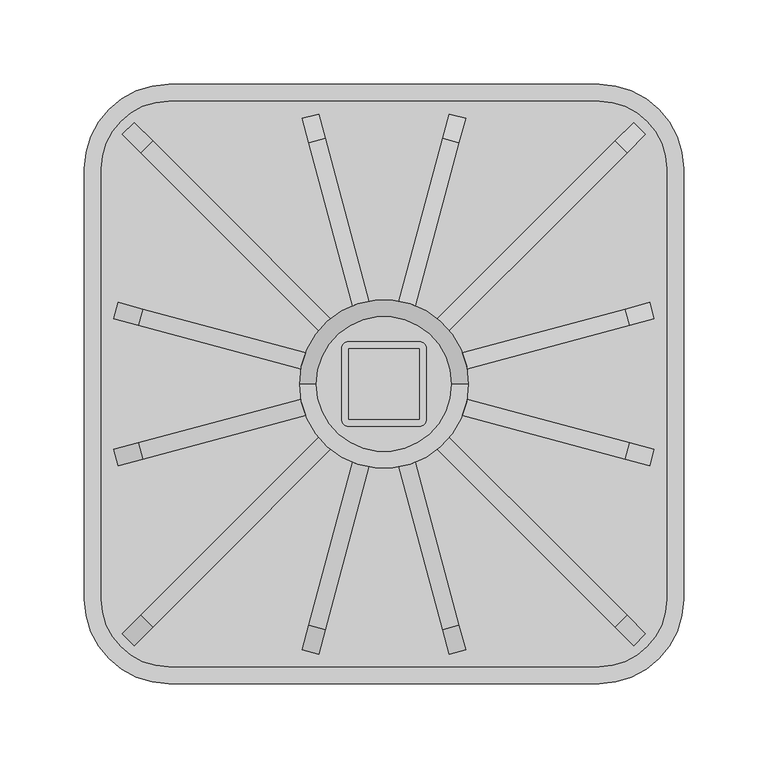
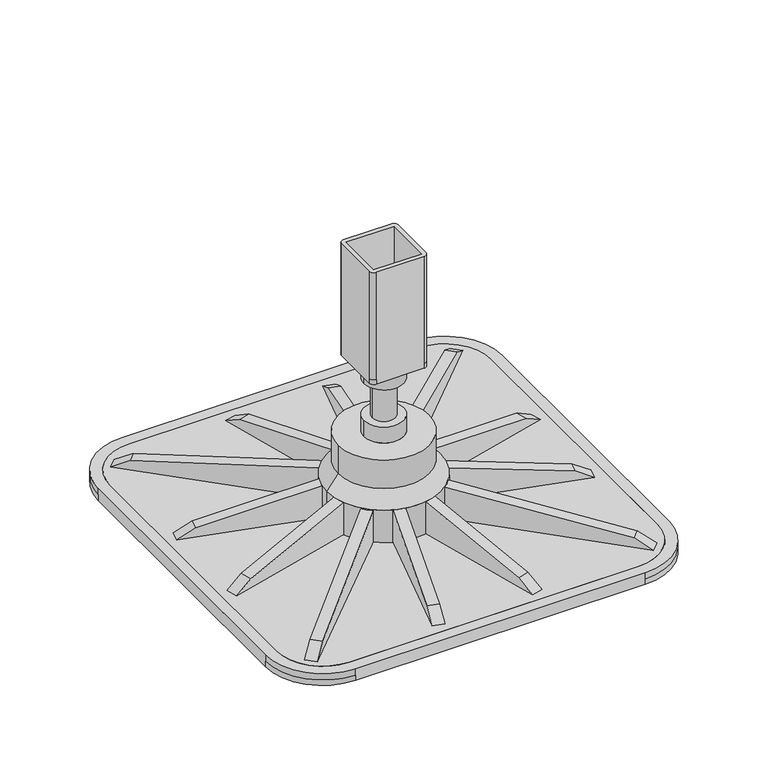
"""IFC4 building model written with IfcOpenShell, lengths in millimetres: proxy geometry, TN_Кровельная опора ТехноНИКОЛЬ : Кровельная опора ТехноНИКОЛЬ 355х355мм с вертикальным кронштейном."""

from ifc_helpers import new_model, si_unit, point, frame, frame_2d, origin, origin_2d, place, context, project, spatial, polyline, circle_curve, trimmed, segment, composite_curve, outline, extrude, source, transform, mapped, element, save
from ifc_brep_helpers import plane_surface, cylinder_surface, revolved_surface, advanced_brep


def generic_models_a60a2459(model_context):
    return source(origin(), model_context, "Body", "SolidModel", [
        extrude(outline(polyline([(214.1306058, 0.0), (198.8913097, -8.6706701), (0.0, -35.5445162), (0.0, 0.0), (214.1306058, 0.0)])), frame((-3.5355339, -3.5355339, 11.0), z_axis=(0.7071067811865469, 0.7071067811865482, 0.0), x_axis=(0.7071067811865482, -0.7071067811865469, 0.0)), (0.0, 0.0, 1.0), 10.0),
        extrude(outline(polyline([(0.0, 0.0), (17.5333016, 1e-07), (203.6920691, -74.9991329), (186.1143887, -105.8931094), (0.0, 0.0)])), frame((154.9487373, 147.8776695, 11.0), z_axis=(-0.707106781186547, 0.7071067811865481, 0.0), x_axis=(-0.6145910150795418, -0.6145910150795407, 0.49452580151797754)), (0.0, 0.0, 1.0), 10.0),
        extrude(outline(polyline([(-214.1306058, 0.0), (0.0, 0.0), (0.0, -35.5445162), (-198.8913097, -8.6706701), (-214.1306058, 0.0)])), frame((-3.5355339, -3.5355339, 11.0), z_axis=(0.7071067811865469, 0.7071067811865482, 0.0), x_axis=(0.7071067811865482, -0.7071067811865469, 0.0)), (0.0, 0.0, 1.0), 10.0),
        extrude(outline(polyline([(0.0, 0.0), (-142.9576707, -80.9713708), (-162.6162897, -46.2634197), (-17.1780129, 0.0), (0.0, 0.0)])), frame((-38.6654497, -159.9920884, 11.0), z_axis=(-0.9659258262890678, 0.25881904510252296, 0.0), x_axis=(-0.22520396734385073, -0.8404726481933256, -0.4928376007687403)), (0.0, 0.0, 1.0), 10.0),
        extrude(outline(polyline([(164.4678969, 0.0), (149.5209418, -8.4659707), (0.1716447, -39.8886346), (0.1716447, 0.0), (164.4678969, 0.0)])), frame((-3.9019744, -1.1282992, 11.0), z_axis=(0.9659258262890678, 0.25881904510252296, 0.0), x_axis=(0.25881904510252296, -0.9659258262890678, 0.0)), (0.0, 0.0, 1.0), 10.0),
        extrude(outline(polyline([(0.0, 0.0), (17.1780129, 0.0), (162.6162896, -46.2634196), (142.9576706, -80.9713707), (0.0, 0.0)])), frame((157.4038979, -48.3247079, 11.0), z_axis=(0.2588190451025272, 0.9659258262890665, 0.0), x_axis=(-0.8404726481933232, 0.22520396734385406, 0.4928376007687429)), (0.0, 0.0, 1.0), 10.0),
        extrude(outline(polyline([(164.4678969, 0.0), (149.5209418, -8.4659707), (0.1716447, -39.8886346), (0.1716447, 0.0), (164.4678969, 0.0)])), frame((1.1282992, -3.9019744, 11.0), z_axis=(-0.25881904510252723, 0.9659258262890665, 0.0), x_axis=(0.9659258262890665, 0.25881904510252723, 0.0)), (0.0, 0.0, 1.0), 10.0),
        extrude(outline(polyline([(0.0, 0.0), (17.1780129, 0.0), (162.6162896, -46.2634196), (142.9576706, -80.9713707), (0.0, 0.0)])), frame((48.3247079, 157.4038979, 11.0), z_axis=(-0.9659258262890661, 0.2588190451025289, 0.0), x_axis=(-0.22520396734385595, -0.8404726481933242, 0.4928376007687402)), (0.0, 0.0, 1.0), 10.0),
        extrude(outline(polyline([(-164.4678969, 0.0), (-0.1716447, 0.0), (-0.1716447, -39.8886346), (-149.5209418, -8.4659707), (-164.4678969, 0.0)])), frame((-5.7572839, -1.4598913, 11.0), z_axis=(0.9659258262890661, 0.25881904510252896, 0.0), x_axis=(0.25881904510252896, -0.9659258262890661, 0.0)), (0.0, 0.0, 1.0), 10.0),
        extrude(outline(polyline([(0.0, 0.0), (-142.9576707, -80.9713708), (-162.6162897, -46.2634197), (-17.1780129, 0.0), (0.0, 0.0)])), frame((-159.9920884, 38.6654497, 11.0), z_axis=(0.25881904510253323, 0.9659258262890649, 0.0), x_axis=(-0.8404726481933251, 0.2252039673438602, -0.4928376007687367)), (0.0, 0.0, 1.0), 10.0),
        extrude(outline(composite_curve([segment(trimmed(circle_curve(origin_2d(), 17.25), [point((-17.25, 0.0))], [point((17.25, 0.0))], False, "CARTESIAN"), True, "CONTINUOUS"), segment(trimmed(circle_curve(origin_2d(), 17.25), [point((17.25, 0.0))], [point((-17.25, 0.0))], False, "CARTESIAN"), True, "CONTINUOUS")], self_intersect=False)), frame((0.0, 0.0, 130.0), z_axis=(0.0, 0.0, 1.0), x_axis=(1.0, 0.0, 0.0)), (0.0, 0.0, 1.0), 16.0),
        advanced_brep(
        [(-21.0, 21.0, 150.0), (-21.0, -21.0, 150.0), (21.0, -21.0, 150.0), (21.0, 21.0, 150.0), (-25.0, 21.0, 146.0), (-21.0, 25.0, 146.0), (21.0, 25.0, 146.0), (25.0, 21.0, 146.0), (25.0, -21.0, 146.0), (21.0, -25.0, 146.0), (-21.0, -25.0, 146.0), (-25.0, -21.0, 146.0), (-25.0, -21.0, 150.0), (-25.0, -21.0, 250.0), (-25.0, 21.0, 250.0), (-25.0, 21.0, 150.0), (-21.0, -25.0, 150.0), (21.0, -25.0, 150.0), (21.0, -25.0, 250.0), (-21.0, -25.0, 250.0), (25.0, -21.0, 150.0), (25.0, 21.0, 150.0), (25.0, 21.0, 250.0), (25.0, -21.0, 250.0), (21.0, 25.0, 150.0), (-21.0, 25.0, 150.0), (-21.0, 25.0, 250.0), (21.0, 25.0, 250.0), (-21.0, -21.0, 250.0), (-21.0, 21.0, 250.0), (21.0, 21.0, 250.0), (21.0, -21.0, 250.0)],
        [
            (0, 1),
            (1, 2),
            (2, 3),
            (3, 0),
            (4, 5, circle_curve(frame((-21.0, 21.0, 146.0), z_axis=(0.0, 0.0, -1.0), x_axis=(1.0, 0.0, 0.0)), 4.0)),
            (5, 6),
            (6, 7, circle_curve(frame((21.0, 21.0, 146.0), z_axis=(0.0, 0.0, -1.0), x_axis=(1.0, 0.0, 0.0)), 4.0)),
            (7, 8),
            (8, 9, circle_curve(frame((21.0, -21.0, 146.0), z_axis=(0.0, 0.0, -1.0), x_axis=(1.0, 0.0, 0.0)), 4.0)),
            (9, 10),
            (10, 11, circle_curve(frame((-21.0, -21.0, 146.0), z_axis=(0.0, 0.0, -1.0), x_axis=(1.0, 0.0, 0.0)), 4.0)),
            (11, 4),
            (11, 12),
            (12, 13),
            (13, 14),
            (14, 15),
            (15, 4),
            (10, 16),
            (16, 12, circle_curve(frame((-21.0, -21.0, 150.0), z_axis=(0.0, 0.0, -1.0), x_axis=(1.0, 0.0, 0.0)), 4.0)),
            (9, 17),
            (17, 18),
            (18, 19),
            (19, 16),
            (8, 20),
            (20, 17, circle_curve(frame((21.0, -21.0, 150.0), z_axis=(0.0, 0.0, -1.0), x_axis=(1.0, 0.0, 0.0)), 4.0)),
            (7, 21),
            (21, 22),
            (22, 23),
            (23, 20),
            (6, 24),
            (24, 21, circle_curve(frame((21.0, 21.0, 150.0), z_axis=(0.0, 0.0, -1.0), x_axis=(1.0, 0.0, 0.0)), 4.0)),
            (5, 25),
            (25, 26),
            (26, 27),
            (27, 24),
            (15, 25, circle_curve(frame((-21.0, 21.0, 150.0), z_axis=(0.0, 0.0, -1.0), x_axis=(1.0, 0.0, 0.0)), 4.0)),
            (26, 14, circle_curve(frame((-21.0, 21.0, 250.0), z_axis=(0.0, 0.0, 1.0), x_axis=(1.0, 0.0, 0.0)), 4.0)),
            (13, 19, circle_curve(frame((-21.0, -21.0, 250.0), z_axis=(0.0, 0.0, 1.0), x_axis=(1.0, 0.0, 0.0)), 4.0)),
            (18, 23, circle_curve(frame((21.0, -21.0, 250.0), z_axis=(0.0, 0.0, 1.0), x_axis=(1.0, 0.0, 0.0)), 4.0)),
            (22, 27, circle_curve(frame((21.0, 21.0, 250.0), z_axis=(0.0, 0.0, 1.0), x_axis=(1.0, 0.0, 0.0)), 4.0)),
            (28, 29),
            (29, 30),
            (30, 31),
            (31, 28),
            (28, 1),
            (0, 29),
            (3, 30),
            (2, 31),
        ],
        [
            plane_surface(frame((-25.0, 21.0, 150.0), z_axis=(0.0, 0.0, 1.0), x_axis=(0.0, -1.0, 0.0))),
            plane_surface(frame((-25.0, 21.0, 146.0), z_axis=(0.0, 0.0, -1.0), x_axis=(0.0, 1.0, 0.0))),
            plane_surface(frame((-25.0, 21.0, 150.0), z_axis=(-1.0, 0.0, 0.0), x_axis=(0.0, 0.0, -1.0))),
            cylinder_surface(frame((-21.0, -21.0, 146.0), z_axis=(0.0, 0.0, 1.0), x_axis=(1.0, 0.0, 0.0)), 4.0),
            plane_surface(frame((-21.0, -25.0, 150.0), z_axis=(0.0, -1.0, 0.0), x_axis=(0.0, 0.0, -1.0))),
            cylinder_surface(frame((21.0, -21.0, 146.0), z_axis=(0.0, 0.0, 1.0), x_axis=(1.0, 0.0, 0.0)), 4.0),
            plane_surface(frame((25.0, -21.0, 150.0), z_axis=(1.0, 0.0, 0.0), x_axis=(0.0, 0.0, -1.0))),
            cylinder_surface(frame((21.0, 21.0, 146.0), z_axis=(0.0, 0.0, 1.0), x_axis=(1.0, 0.0, 0.0)), 4.0),
            plane_surface(frame((21.0, 25.0, 150.0), z_axis=(0.0, 1.0, 0.0), x_axis=(0.0, 0.0, -1.0))),
            cylinder_surface(frame((-21.0, 21.0, 146.0), z_axis=(0.0, 0.0, 1.0), x_axis=(1.0, 0.0, 0.0)), 4.0),
            plane_surface(frame((-25.0, 25.0, 250.0), z_axis=(0.0, 0.0, 1.0), x_axis=(-1.0, 0.0, 0.0))),
            plane_surface(frame((-21.0, -21.0, 250.0), z_axis=(1.0, 0.0, 0.0), x_axis=(0.0, 0.0, -1.0))),
            plane_surface(frame((-21.0, 21.0, 250.0), z_axis=(0.0, -1.0, 0.0), x_axis=(0.0, 0.0, -1.0))),
            plane_surface(frame((21.0, 21.0, 250.0), z_axis=(-1.0, 0.0, 0.0), x_axis=(0.0, 0.0, -1.0))),
            plane_surface(frame((21.0, -21.0, 250.0), z_axis=(0.0, 1.0, 0.0), x_axis=(0.0, 0.0, -1.0))),
        ],
        [
            (0, [[1, 2, 3, 4]]),
            (1, [[5, 6, 7, 8, 9, 10, 11, 12]]),
            (2, [[-12, 13, 14, 15, 16, 17]]),
            (3, [[-11, 18, 19, -13]]),
            (4, [[-10, 20, 21, 22, 23, -18]]),
            (5, [[-9, 24, 25, -20]]),
            (6, [[-8, 26, 27, 28, 29, -24]]),
            (7, [[-7, 30, 31, -26]]),
            (8, [[-6, 32, 33, 34, 35, -30]]),
            (9, [[-5, -17, 36, -32]]),
            (10, [[-34, 37, -15, 38, -22, 39, -28, 40], [41, 42, 43, 44]]),
            (9, [[-37, -33, -36, -16]]),
            (3, [[-38, -14, -19, -23]]),
            (5, [[-39, -21, -25, -29]]),
            (7, [[-40, -27, -31, -35]]),
            (11, [[-41, 45, -1, 46]]),
            (12, [[-42, -46, -4, 47]]),
            (13, [[-43, -47, -3, 48]]),
            (14, [[-44, -48, -2, -45]]),
        ],
    ),
        advanced_brep(
        [(-40.0, 0.0, 80.6), (40.0, 0.0, 80.6), (17.25, 0.0, 80.6), (-17.25, 0.0, 80.6), (-40.0, 0.0, 54.2), (40.0, 0.0, 54.2), (-10.0, 0.0, 146.0), (10.0, 0.0, 146.0), (-10.0, 0.0, 95.6), (10.0, 0.0, 95.6), (-17.25, 0.0, 95.6), (17.25, 0.0, 95.6)],
        [
            (0, 1, circle_curve(frame((0.0, 0.0, 80.6), z_axis=(0.0, 0.0, 1.0), x_axis=(1.0, 0.0, 0.0)), 40.0)),
            (1, 0, circle_curve(frame((0.0, 0.0, 80.6), z_axis=(0.0, 0.0, 1.0), x_axis=(1.0, 0.0, 0.0)), 40.0)),
            (2, 3, circle_curve(frame((0.0, 0.0, 80.6), z_axis=(0.0, 0.0, -1.0), x_axis=(1.0, 0.0, 0.0)), 17.25)),
            (3, 2, circle_curve(frame((0.0, 0.0, 80.6), z_axis=(0.0, 0.0, -1.0), x_axis=(1.0, 0.0, 0.0)), 17.25)),
            (4, 5, circle_curve(frame((0.0, 0.0, 54.2), z_axis=(0.0, 0.0, -1.0), x_axis=(1.0, 0.0, 0.0)), 40.0)),
            (5, 4, circle_curve(frame((0.0, 0.0, 54.2), z_axis=(0.0, 0.0, -1.0), x_axis=(1.0, 0.0, 0.0)), 40.0)),
            (0, 4),
            (5, 1),
            (6, 7, circle_curve(frame((0.0, 0.0, 146.0), z_axis=(0.0, 0.0, 1.0), x_axis=(1.0, 0.0, 0.0)), 10.0)),
            (7, 6, circle_curve(frame((0.0, 0.0, 146.0), z_axis=(0.0, 0.0, 1.0), x_axis=(1.0, 0.0, 0.0)), 10.0)),
            (6, 8),
            (8, 9, circle_curve(frame((0.0, 0.0, 95.6), z_axis=(0.0, 0.0, 1.0), x_axis=(1.0, 0.0, 0.0)), 10.0)),
            (9, 7),
            (9, 8, circle_curve(frame((0.0, 0.0, 95.6), z_axis=(0.0, 0.0, 1.0), x_axis=(1.0, 0.0, 0.0)), 10.0)),
            (10, 11, circle_curve(frame((0.0, 0.0, 95.6), z_axis=(0.0, 0.0, 1.0), x_axis=(1.0, 0.0, 0.0)), 17.25)),
            (11, 10, circle_curve(frame((0.0, 0.0, 95.6), z_axis=(0.0, 0.0, 1.0), x_axis=(1.0, 0.0, 0.0)), 17.25)),
            (10, 3),
            (2, 11),
        ],
        [
            plane_surface(frame((40.0, 0.0, 80.6), z_axis=(0.0, 0.0, 1.0), x_axis=(0.0, 1.0, 0.0))),
            plane_surface(frame((40.0, 0.0, 54.2), z_axis=(0.0, 0.0, -1.0), x_axis=(0.0, -1.0, 0.0))),
            cylinder_surface(frame((0.0, 0.0, 54.2), z_axis=(0.0, 0.0, 1.0), x_axis=(1.0, 0.0, 0.0)), 40.0),
            plane_surface(frame((10.0, 0.0, 146.0), z_axis=(0.0, 0.0, 1.0), x_axis=(0.0, 1.0, 0.0))),
            cylinder_surface(frame((0.0, 0.0, 80.6), z_axis=(0.0, 0.0, 1.0), x_axis=(1.0, 0.0, 0.0)), 10.0),
            plane_surface(frame((17.25, 0.0, 95.6), z_axis=(0.0, 0.0, 1.0), x_axis=(0.0, 1.0, 0.0))),
            cylinder_surface(frame((0.0, 0.0, 80.6), z_axis=(0.0, 0.0, 1.0), x_axis=(1.0, 0.0, 0.0)), 17.25),
        ],
        [
            (0, [[1, 2], [3, 4]]),
            (1, [[5, 6]]),
            (2, [[-1, 7, -6, 8]]),
            (2, [[-2, -8, -5, -7]]),
            (3, [[9, 10]]),
            (4, [[-9, 11, 12, 13]]),
            (4, [[-10, -13, 14, -11]]),
            (5, [[15, 16], [-12, -14]]),
            (6, [[-15, 17, -3, 18]]),
            (6, [[-16, -18, -4, -17]]),
        ],
    ),
        extrude(outline(polyline([(-164.4678969, 0.0), (-0.1716447, 0.0), (-0.1716447, -39.8886346), (-149.5209418, -8.4659707), (-164.4678969, 0.0)])), frame((1.4598913, -5.7572839, 11.0), z_axis=(-0.25881904510253323, 0.965925826289065, 0.0), x_axis=(0.965925826289065, 0.25881904510253323, 0.0)), (0.0, 0.0, 1.0), 10.0),
        extrude(outline(polyline([(0.0, 0.0), (-186.1143887, -105.8931094), (-203.6920691, -74.9991329), (-17.5333016, 1e-07), (0.0, 0.0)])), frame((-147.8776695, -154.9487373, 11.0), z_axis=(-0.7071067811865469, 0.7071067811865482, 0.0), x_axis=(-0.6145910150795192, -0.6145910150795181, -0.4945258015180338)), (0.0, 0.0, 1.0), 10.0),
        advanced_brep(
        [(-40.0, 0.0, 54.2), (40.0, 0.0, 54.2), (-50.0, 0.0, 41.0), (50.0, 0.0, 41.0)],
        [
            (0, 1, circle_curve(frame((0.0, 0.0, 54.2), z_axis=(0.0, 0.0, 1.0), x_axis=(-1.0, 0.0, 0.0)), 40.0)),
            (1, 0, circle_curve(frame((0.0, 0.0, 54.2), z_axis=(0.0, 0.0, 1.0), x_axis=(1.0, 0.0, 0.0)), 40.0)),
            (2, 3, circle_curve(frame((0.0, 0.0, 41.0), z_axis=(0.0, 0.0, -1.0), x_axis=(1.0, 0.0, 0.0)), 50.0)),
            (3, 2, circle_curve(frame((0.0, 0.0, 41.0), z_axis=(0.0, 0.0, -1.0), x_axis=(-1.0, 0.0, 0.0)), 50.0)),
            (3, 1),
            (0, 2),
        ],
        [
            plane_surface(frame((0.0, 0.0, 54.2), z_axis=(0.0, 0.0, 1.0), x_axis=(0.0, -1.0, 0.0))),
            plane_surface(frame((0.0, 0.0, 41.0), z_axis=(0.0, 0.0, -1.0), x_axis=(0.0, -1.0, 0.0))),
            revolved_surface(polyline([(-40.0, 0.0, 54.2), (-50.0, 0.0, 41.0)]), (0.0, 0.0, 107.0), (0.0, 0.0, -1.0)),
            revolved_surface(polyline([(40.0, 0.0, 54.2), (50.0, 0.0, 41.0)]), (0.0, 0.0, 107.0), (0.0, 0.0, -1.0)),
        ],
        [
            (0, [[1, 2]]),
            (1, [[3, 4]]),
            (2, [[-4, 5, -1, 6]]),
            (3, [[-3, -6, -2, -5]]),
        ],
    ),
        extrude(outline(composite_curve([segment(trimmed(circle_curve(origin_2d(), 50.0), [point((-50.0, 0.0))], [point((50.0, 0.0))], False, "CARTESIAN"), True, "CONTINUOUS"), segment(trimmed(circle_curve(origin_2d(), 50.0), [point((50.0, 0.0))], [point((-50.0, 0.0))], False, "CARTESIAN"), True, "CONTINUOUS")], self_intersect=False)), frame((0.0, 0.0, 11.0), z_axis=(0.0, 0.0, 1.0), x_axis=(1.0, 0.0, 0.0)), (0.0, 0.0, 1.0), 30.0),
        extrude(outline(composite_curve([segment(trimmed(circle_curve(frame_2d((127.5, 127.5)), 40.0), [point((127.5, 167.5))], [point((167.5, 127.5))], False, "CARTESIAN"), True, "CONTINUOUS"), segment(polyline([(167.5, 127.5), (167.5, -127.5)]), True, "CONTINUOUS"), segment(trimmed(circle_curve(frame_2d((127.5, -127.5)), 40.0), [point((167.5, -127.5))], [point((127.5, -167.5))], False, "CARTESIAN"), True, "CONTINUOUS"), segment(polyline([(127.5, -167.5), (-127.5, -167.5)]), True, "CONTINUOUS"), segment(trimmed(circle_curve(frame_2d((-127.5, -127.5)), 40.0), [point((-127.5, -167.5))], [point((-167.5, -127.5))], False, "CARTESIAN"), True, "CONTINUOUS"), segment(polyline([(-167.5, -127.5), (-167.5, 127.5)]), True, "CONTINUOUS"), segment(trimmed(circle_curve(frame_2d((-127.5, 127.5)), 40.0), [point((-167.5, 127.5))], [point((-127.5, 167.5))], False, "CARTESIAN"), True, "CONTINUOUS"), segment(polyline([(-127.5, 167.5), (127.5, 167.5)]), True, "CONTINUOUS")], self_intersect=False)), frame((0.0, 0.0, 5.0), z_axis=(0.0, 0.0, 1.0), x_axis=(1.0, 0.0, 0.0)), (0.0, 0.0, 1.0), 6.0),
        advanced_brep(
        [(-127.5, 167.5, 5.0), (-167.5, 127.5, 5.0), (-167.5, -127.5, 5.0), (-127.5, -167.5, 5.0), (127.5, -167.5, 5.0), (167.5, -127.5, 5.0), (167.5, 127.5, 5.0), (127.5, 167.5, 5.0), (-177.5, -127.5, 0.0), (-177.5, 127.5, 0.0), (-127.5, 177.5, 0.0), (127.5, 177.5, 0.0), (177.5, 127.5, 0.0), (177.5, -127.5, 0.0), (127.5, -177.5, 0.0), (-127.5, -177.5, 0.0), (-127.5, -177.5, 5.0), (-177.5, -127.5, 5.0), (127.5, -177.5, 5.0), (127.5, -177.5, 11.0), (-127.5, -177.5, 11.0), (177.5, -127.5, 5.0), (177.5, 127.5, 5.0), (177.5, 127.5, 11.0), (177.5, -127.5, 11.0), (127.5, 177.5, 5.0), (-127.5, 177.5, 5.0), (-127.5, 177.5, 11.0), (127.5, 177.5, 11.0), (-177.5, 127.5, 5.0), (-177.5, -127.5, 11.0), (-177.5, 127.5, 11.0), (-167.5, 127.5, 11.0), (-127.5, 167.5, 11.0), (127.5, 167.5, 11.0), (167.5, 127.5, 11.0), (167.5, -127.5, 11.0), (127.5, -167.5, 11.0), (-127.5, -167.5, 11.0), (-167.5, -127.5, 11.0)],
        [
            (0, 1, circle_curve(frame((-127.5, 127.5, 5.0), z_axis=(0.0, 0.0, 1.0), x_axis=(1.0, 0.0, 0.0)), 40.0)),
            (1, 2),
            (2, 3, circle_curve(frame((-127.5, -127.5, 5.0), z_axis=(0.0, 0.0, 1.0), x_axis=(1.0, 0.0, 0.0)), 40.0)),
            (3, 4),
            (4, 5, circle_curve(frame((127.5, -127.5, 5.0), z_axis=(0.0, 0.0, 1.0), x_axis=(1.0, 0.0, 0.0)), 40.0)),
            (5, 6),
            (6, 7, circle_curve(frame((127.5, 127.5, 5.0), z_axis=(0.0, 0.0, 1.0), x_axis=(1.0, 0.0, 0.0)), 40.0)),
            (7, 0),
            (8, 9),
            (9, 10, circle_curve(frame((-127.5, 127.5, 0.0), z_axis=(0.0, 0.0, -1.0), x_axis=(1.0, 0.0, 0.0)), 50.0)),
            (10, 11),
            (11, 12, circle_curve(frame((127.5, 127.5, 0.0), z_axis=(0.0, 0.0, -1.0), x_axis=(1.0, 0.0, 0.0)), 50.0)),
            (12, 13),
            (13, 14, circle_curve(frame((127.5, -127.5, 0.0), z_axis=(0.0, 0.0, -1.0), x_axis=(1.0, 0.0, 0.0)), 50.0)),
            (14, 15),
            (15, 8, circle_curve(frame((-127.5, -127.5, 0.0), z_axis=(0.0, 0.0, -1.0), x_axis=(1.0, 0.0, 0.0)), 50.0)),
            (15, 16),
            (16, 17, circle_curve(frame((-127.5, -127.5, 5.0), z_axis=(0.0, 0.0, -1.0), x_axis=(1.0, 0.0, 0.0)), 50.0)),
            (17, 8),
            (14, 18),
            (18, 19),
            (19, 20),
            (20, 16),
            (13, 21),
            (21, 18, circle_curve(frame((127.5, -127.5, 5.0), z_axis=(0.0, 0.0, -1.0), x_axis=(1.0, 0.0, 0.0)), 50.0)),
            (12, 22),
            (22, 23),
            (23, 24),
            (24, 21),
            (11, 25),
            (25, 22, circle_curve(frame((127.5, 127.5, 5.0), z_axis=(0.0, 0.0, -1.0), x_axis=(1.0, 0.0, 0.0)), 50.0)),
            (10, 26),
            (26, 27),
            (27, 28),
            (28, 25),
            (9, 29),
            (29, 26, circle_curve(frame((-127.5, 127.5, 5.0), z_axis=(0.0, 0.0, -1.0), x_axis=(1.0, 0.0, 0.0)), 50.0)),
            (17, 30),
            (30, 31),
            (31, 29),
            (27, 31, circle_curve(frame((-127.5, 127.5, 11.0), z_axis=(0.0, 0.0, 1.0), x_axis=(1.0, 0.0, 0.0)), 50.0)),
            (30, 20, circle_curve(frame((-127.5, -127.5, 11.0), z_axis=(0.0, 0.0, 1.0), x_axis=(1.0, 0.0, 0.0)), 50.0)),
            (19, 24, circle_curve(frame((127.5, -127.5, 11.0), z_axis=(0.0, 0.0, 1.0), x_axis=(1.0, 0.0, 0.0)), 50.0)),
            (23, 28, circle_curve(frame((127.5, 127.5, 11.0), z_axis=(0.0, 0.0, 1.0), x_axis=(1.0, 0.0, 0.0)), 50.0)),
            (32, 33, circle_curve(frame((-127.5, 127.5, 11.0), z_axis=(0.0, 0.0, -1.0), x_axis=(1.0, 0.0, 0.0)), 40.0)),
            (33, 34),
            (34, 35, circle_curve(frame((127.5, 127.5, 11.0), z_axis=(0.0, 0.0, -1.0), x_axis=(1.0, 0.0, 0.0)), 40.0)),
            (35, 36),
            (36, 37, circle_curve(frame((127.5, -127.5, 11.0), z_axis=(0.0, 0.0, -1.0), x_axis=(1.0, 0.0, 0.0)), 40.0)),
            (37, 38),
            (38, 39, circle_curve(frame((-127.5, -127.5, 11.0), z_axis=(0.0, 0.0, -1.0), x_axis=(1.0, 0.0, 0.0)), 40.0)),
            (39, 32),
            (32, 1),
            (0, 33),
            (7, 34),
            (6, 35),
            (5, 36),
            (4, 37),
            (3, 38),
            (2, 39),
        ],
        [
            plane_surface(frame((-77.5, -127.5, 5.0), z_axis=(0.0, 0.0, 1.0), x_axis=(0.0, 1.0, 0.0))),
            plane_surface(frame((-77.5, -127.5, 0.0), z_axis=(0.0, 0.0, -1.0), x_axis=(0.0, -1.0, 0.0))),
            cylinder_surface(frame((-127.5, -127.5, 0.0), z_axis=(0.0, 0.0, 1.0), x_axis=(1.0, 0.0, 0.0)), 50.0),
            plane_surface(frame((-127.5, -177.5, 5.0), z_axis=(0.0, -1.0, 0.0), x_axis=(0.0, 0.0, -1.0))),
            cylinder_surface(frame((127.5, -127.5, 0.0), z_axis=(0.0, 0.0, 1.0), x_axis=(1.0, 0.0, 0.0)), 50.0),
            plane_surface(frame((177.5, -127.5, 5.0), z_axis=(1.0, 0.0, 0.0), x_axis=(0.0, 0.0, -1.0))),
            cylinder_surface(frame((127.5, 127.5, 0.0), z_axis=(0.0, 0.0, 1.0), x_axis=(1.0, 0.0, 0.0)), 50.0),
            plane_surface(frame((127.5, 177.5, 5.0), z_axis=(0.0, 1.0, 0.0), x_axis=(0.0, 0.0, -1.0))),
            cylinder_surface(frame((-127.5, 127.5, 0.0), z_axis=(0.0, 0.0, 1.0), x_axis=(1.0, 0.0, 0.0)), 50.0),
            plane_surface(frame((-177.5, 127.5, 5.0), z_axis=(-1.0, 0.0, 0.0), x_axis=(0.0, 0.0, -1.0))),
            plane_surface(frame((-77.5, 127.5, 11.0), z_axis=(0.0, 0.0, 1.0), x_axis=(0.0, 1.0, 0.0))),
            cylinder_surface(frame((-127.5, 127.5, 5.0), z_axis=(0.0, 0.0, 1.0), x_axis=(1.0, 0.0, 0.0)), 50.0),
            cylinder_surface(frame((-127.5, -127.5, 5.0), z_axis=(0.0, 0.0, 1.0), x_axis=(1.0, 0.0, 0.0)), 50.0),
            cylinder_surface(frame((127.5, -127.5, 5.0), z_axis=(0.0, 0.0, 1.0), x_axis=(1.0, 0.0, 0.0)), 50.0),
            cylinder_surface(frame((127.5, 127.5, 5.0), z_axis=(0.0, 0.0, 1.0), x_axis=(1.0, 0.0, 0.0)), 50.0),
            revolved_surface(polyline([(-87.5, 127.5, 5.0), (-87.5, 127.5, 11.0)]), (-127.5, 127.5, 0.0), (0.0, 0.0, -1.0)),
            plane_surface(frame((-127.5, 167.5, 11.0), z_axis=(0.0, -1.0, 0.0), x_axis=(0.0, 0.0, -1.0))),
            revolved_surface(polyline([(167.5, 127.5, 5.0), (167.5, 127.5, 11.0)]), (127.5, 127.5, 0.0), (0.0, 0.0, -1.0)),
            plane_surface(frame((167.5, 127.5, 11.0), z_axis=(-1.0, 0.0, 0.0), x_axis=(0.0, 0.0, -1.0))),
            revolved_surface(polyline([(167.5, -127.5, 5.0), (167.5, -127.5, 11.0)]), (127.5, -127.5, 0.0), (0.0, 0.0, -1.0)),
            plane_surface(frame((127.5, -167.5, 11.0), z_axis=(0.0, 1.0, 0.0), x_axis=(0.0, 0.0, -1.0))),
            revolved_surface(polyline([(-87.5, -127.5, 5.0), (-87.5, -127.5, 11.0)]), (-127.5, -127.5, 0.0), (0.0, 0.0, -1.0)),
            plane_surface(frame((-167.5, -127.5, 11.0), z_axis=(1.0, 0.0, 0.0), x_axis=(0.0, 0.0, -1.0))),
        ],
        [
            (0, [[1, 2, 3, 4, 5, 6, 7, 8]]),
            (1, [[9, 10, 11, 12, 13, 14, 15, 16]]),
            (2, [[-16, 17, 18, 19]]),
            (3, [[-15, 20, 21, 22, 23, -17]]),
            (4, [[-14, 24, 25, -20]]),
            (5, [[-13, 26, 27, 28, 29, -24]]),
            (6, [[-12, 30, 31, -26]]),
            (7, [[-11, 32, 33, 34, 35, -30]]),
            (8, [[-10, 36, 37, -32]]),
            (9, [[-9, -19, 38, 39, 40, -36]]),
            (10, [[41, -39, 42, -22, 43, -28, 44, -34], [45, 46, 47, 48, 49, 50, 51, 52]]),
            (11, [[-41, -33, -37, -40]]),
            (12, [[-42, -38, -18, -23]]),
            (13, [[-43, -21, -25, -29]]),
            (14, [[-44, -27, -31, -35]]),
            (15, [[-45, 53, -1, 54]]),
            (16, [[-46, -54, -8, 55]]),
            (17, [[-47, -55, -7, 56]]),
            (18, [[-48, -56, -6, 57]]),
            (19, [[-49, -57, -5, 58]]),
            (20, [[-50, -58, -4, 59]]),
            (21, [[-51, -59, -3, 60]]),
            (22, [[-52, -60, -2, -53]]),
        ],
    ),
    ])


if __name__ == "__main__":
    model = new_model("IFC4")
    model_context = context("Model", 3, world=origin())
    ifc_project = project(units=[si_unit("LENGTHUNIT", "METRE", prefix="MILLI")], contexts=[model_context])
    site = spatial("IfcSite", under=ifc_project)
    building = spatial("IfcBuilding", under=site)
    placement = place(None, origin())
    generic_models_shape = generic_models_a60a2459(model_context)
    element("IfcBuildingElementProxy", 1, Name="TN_Кровельная опора ТехноНИКОЛЬ : Кровельная опора ТехноНИКОЛЬ 355х355мм с вертикальным кронштейном", ObjectType="TN_Кровельная опора ТехноНИКОЛЬ : Кровельная опора ТехноНИКОЛЬ 355х355мм с вертикальным кронштейном", at=placement, inside=building, context=model_context, shape_type="MappedRepresentation", body=[
        mapped(generic_models_shape, transform((0.0, 0.0, 0.0), x_axis=(1.0, 0.0, 0.0), y_axis=(0.0, 1.0, 0.0), z_axis=(0.0, 0.0, 1.0))),
    ])
    save(model, "model.ifc")

# Revit data of these elements
# Type "TN_Кровельная опора ТехноНИКОЛЬ : Кровельная опора ТехноНИКОЛЬ 355х355мм с вертикальным кронштейном"
#   Description = "Кровельные опоры ТехноНИКОЛЬ, служат в качестве решение для размещения инженерных коммуникаций и промышленного оборудования на крыше здания, чиллеров, кондиционеров, воздуховодов, трубопроводов. Отличительной особенностью является регулировка кронштейна опоры, для необходимости компенсации уклона кровли."
#   Manufacturer = "ТехноНИКОЛЬ"
#   ADSK_Обозначение = "ТехноНИКОЛЬ"
#   ADSK_Наименование = "Кровельная опора ТехноНИКОЛЬ 355х355мм с вертикальным кронштейном"
#   ADSK_Масса_Текст = ""
#   ADSK_Марка = "355х355"
#   ADSK_Код изделия = "43362"
#   ADSK_Завод-изготовитель = "ТехноНИКОЛЬ"
#   ADSK_Единица измерения = "шт."
#   ADSK_Группирование = "Комплектующие к опорам"
#   ADSK_URL страницы изделия = ""
#   ADSK_URL документации изделия = ""
#   ADSK_Размер_Ширина = 355 mm
#   ADSK_Масса = 0
#   ADSK_Количество = 1
#   Видимость_Кронштейн горизонтальный = no
#   Видимость_Кронштейн вертикальный = yes
#   ADSK_Материал = TN_Пластик_Красный
#   Default Elevation = 0
#   URL = ""
# Element 1 (IfcBuildingElementProxy, "TN_Кровельная опора ТехноНИКОЛЬ : Кровельная опора ТехноНИКОЛЬ 355х355мм с вертикальным кронштейном")
#   Materials on its faces: "TN_Пластик_Красный", "TN_СтальГальванизированная_Серый", "TN_Пластик_ТемноСерый"
# Materials
#   "TN_Пластик_Красный": class "Типовые", colour RGB 200 10 50, transparency 0, Cost = 0
#   "TN_СтальГальванизированная_Серый": class "Типовые", colour RGB 206 210 213, transparency 0, Cost = 0
#   "TN_Пластик_ТемноСерый": class "Типовые", colour RGB 50 50 50, transparency 0, Cost = 0
